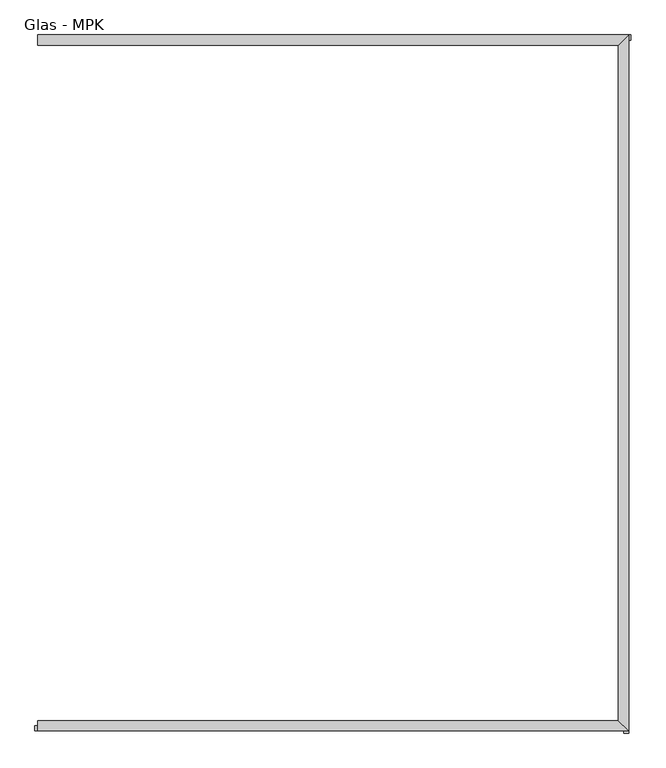
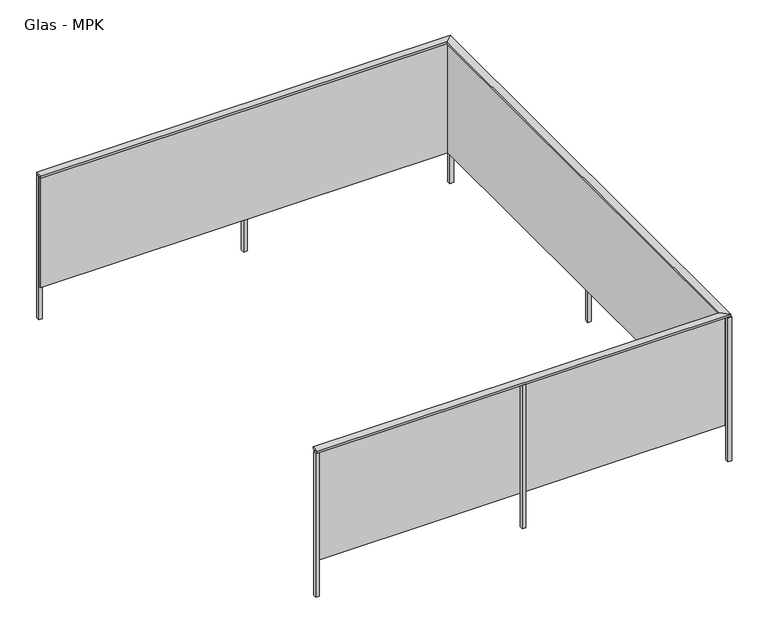
"""IFC4 building model written with IfcOpenShell, lengths in millimetres: railing geometry, Glas - MPK."""

import ifcopenshell
import ifcopenshell.guid

model = None  # the IFC model being written
_history = None  # IfcOwnerHistory: only IFC2X3 demands one
_inside = {}  # id of a spatial element -> (the spatial element, [elements in it])
_under = {}  # id of a project, library or spatial element -> (it, [spatial elements below it])
_declared = {}  # id of a project -> (the project, [libraries it declares])
_typed = {}  # id of a type object -> (the type object, [elements of that type])
_made_of = {}  # id of a material, layer set ... -> (it, [elements and type objects made of it])


def new_model(schema):
    """Start an empty IFC model of exactly this schema.

    Asked for "IFC4X3", IfcOpenShell would pick the latest addendum, in which some entities
    have other attributes; the version numbers below select the first issue.
    IFC2X3 requires an IfcOwnerHistory on every rooted entity: one is made here for all.
    """
    global model, _history
    if schema == "IFC4X3":
        model = ifcopenshell.file(schema_version=(4, 3, 0, 0))
    else:
        model = ifcopenshell.file(schema=schema)
    _inside.clear()
    _under.clear()
    _declared.clear()
    _typed.clear()
    _made_of.clear()
    _history = None
    if model.schema == "IFC2X3":
        org = make("IfcOrganization", Name="unknown")
        user = make(
            "IfcPersonAndOrganization",
            ThePerson=make("IfcPerson", FamilyName="unknown"),
            TheOrganization=org,
        )
        app = make(
            "IfcApplication",
            ApplicationDeveloper=org,
            Version="unknown",
            ApplicationFullName="unknown",
            ApplicationIdentifier="unknown",
        )
        _history = make(
            "IfcOwnerHistory",
            OwningUser=user,
            OwningApplication=app,
            ChangeAction="ADDED",
            CreationDate=0,
        )
    return model


def make(cls, **values):
    """One entity of the class cls with the attributes given. An attribute that is None is left unset."""
    return model.create_entity(
        cls, **{name: value for name, value in values.items() if value is not None}
    )


def rooted(cls, **values):
    """An entity with a GlobalId (a new one), such as an element, a storey or a relation."""
    return make(cls, GlobalId=ifcopenshell.guid.new(), OwnerHistory=_history, **values)


def si_unit(unit_type, name, prefix=None):
    """IfcSIUnit, for example si_unit("LENGTHUNIT", "METRE", prefix="MILLI")."""
    return make("IfcSIUnit", UnitType=unit_type, Prefix=prefix, Name=name)


def assignment(units):
    """IfcUnitAssignment: the units of a project."""
    return None if units is None else make("IfcUnitAssignment", Units=units)


def point(xyz):
    """IfcCartesianPoint."""
    return None if xyz is None else make("IfcCartesianPoint", Coordinates=xyz)


def direction(xyz):
    """IfcDirection."""
    return None if xyz is None else make("IfcDirection", DirectionRatios=xyz)


def frame(location, z_axis=None, x_axis=None):
    """IfcAxis2Placement3D, a coordinate frame: its origin and axes. An axis left out is left unset."""
    return make(
        "IfcAxis2Placement3D",
        Location=point(location),
        Axis=direction(z_axis),
        RefDirection=direction(x_axis),
    )


def origin():
    """The frame at (0, 0, 0) with its axes left unset."""
    return frame((0.0, 0.0, 0.0))


def place(relative_to, where):
    """IfcLocalPlacement: puts the frame where relative to a parent placement (None: the world)."""
    return make(
        "IfcLocalPlacement", PlacementRelTo=relative_to, RelativePlacement=where
    )


def context(
    kind, dimensions, precision=None, world=None, true_north=None, identifier=None
):
    """IfcGeometricRepresentationContext, for example the 3D "Model" context."""
    return make(
        "IfcGeometricRepresentationContext",
        ContextIdentifier=identifier,
        ContextType=kind,
        CoordinateSpaceDimension=dimensions,
        Precision=precision,
        WorldCoordinateSystem=world,
        TrueNorth=true_north,
    )


def project(units=None, contexts=None):
    """IfcProject with its units and contexts."""
    return rooted(
        "IfcProject",
        Name="project",
        RepresentationContexts=contexts,
        UnitsInContext=assignment(units),
    )


def spatial(cls, under=None, at=None, **own):
    """A site, building, storey or space (cls), placed at a placement, below another one or the project."""
    s = rooted(cls, ObjectPlacement=at, **own)
    if under is not None:
        _under.setdefault(under.id(), (under, []))[1].append(s)
    return s


def polyline(points):
    """IfcPolyline through the points."""
    return make("IfcPolyline", Points=[point(p) for p in points])


def outline(outer, holes=None, kind="AREA"):
    """IfcArbitraryClosedProfileDef: a profile drawn as a closed curve; with holes, ...WithVoids."""
    if holes is None:
        return make("IfcArbitraryClosedProfileDef", ProfileType=kind, OuterCurve=outer)
    return make(
        "IfcArbitraryProfileDefWithVoids",
        ProfileType=kind,
        OuterCurve=outer,
        InnerCurves=holes,
    )


def extrude(swept, where, along, depth):
    """IfcExtrudedAreaSolid: the profile swept, set in the frame where, extruded along a direction by depth."""
    return make(
        "IfcExtrudedAreaSolid",
        SweptArea=swept,
        Position=where,
        ExtrudedDirection=direction(along),
        Depth=depth,
    )


def faces_of(points, faces, orient=None, outer=None):
    """IfcFace entities. A face is a list of loops; a loop is a list of indices into points, from 0.

    orient and outer hold one flag for each loop. By default every Orientation is true, the
    first loop of a face is its IfcFaceOuterBound and the others are IfcFaceBound.
    """
    made = []
    for i, loops in enumerate(faces):
        bounds = []
        for j, loop in enumerate(loops):
            is_outer = j == 0 if outer is None else outer[i][j]
            bounds.append(
                make(
                    "IfcFaceOuterBound" if is_outer else "IfcFaceBound",
                    Bound=make("IfcPolyLoop", Polygon=[points[k] for k in loop]),
                    Orientation=True if orient is None else orient[i][j],
                )
            )
        made.append(make("IfcFace", Bounds=bounds))
    return made


def faceted_brep(points, faces, orient=None, outer=None, voids=None):
    """IfcFacetedBrep: a solid bounded by flat faces; with voids (closed shells), ...WithVoids."""
    shared = [point(p) for p in points]
    hull = make("IfcClosedShell", CfsFaces=faces_of(shared, faces, orient, outer))
    if voids is None:
        return make("IfcFacetedBrep", Outer=hull)
    return make(
        "IfcFacetedBrepWithVoids",
        Outer=hull,
        Voids=[
            make(cls, CfsFaces=faces_of(shared, fs, o, b)) for cls, fs, o, b in voids
        ],
    )


def shape(context_of_items, identifier, shape_type, items):
    """IfcShapeRepresentation: the items that make up one representation, for example the "Body"."""
    return make(
        "IfcShapeRepresentation",
        ContextOfItems=context_of_items,
        RepresentationIdentifier=identifier,
        RepresentationType=shape_type,
        Items=items,
    )


def source(mapping_origin, context_of_items, identifier, shape_type, items):
    """IfcRepresentationMap: a shape defined once, which mapped items show again and again."""
    return make(
        "IfcRepresentationMap",
        MappingOrigin=mapping_origin,
        MappedRepresentation=shape(context_of_items, identifier, shape_type, items),
    )


def transform(
    local_origin,
    x_axis=None,
    y_axis=None,
    z_axis=None,
    scale=None,
    scale2=None,
    scale3=None,
    uniform=True,
):
    """IfcCartesianTransformationOperator3D, or its non-uniform kind. x_axis, y_axis, z_axis: its Axis1, 2, 3."""
    if uniform:
        return make(
            "IfcCartesianTransformationOperator3D",
            Axis1=direction(x_axis),
            Axis2=direction(y_axis),
            LocalOrigin=point(local_origin),
            Scale=scale,
            Axis3=direction(z_axis),
        )
    return make(
        "IfcCartesianTransformationOperator3DnonUniform",
        Axis1=direction(x_axis),
        Axis2=direction(y_axis),
        LocalOrigin=point(local_origin),
        Scale=scale,
        Axis3=direction(z_axis),
        Scale2=scale2,
        Scale3=scale3,
    )


def mapped(mapping_source, mapping_target):
    """IfcMappedItem: shows the shape of a source again, moved by a transform."""
    return make(
        "IfcMappedItem", MappingSource=mapping_source, MappingTarget=mapping_target
    )


def made_of(thing, what):
    """Note that an element or type object is made of a material, layer set ...; save() writes the relation."""
    if what is not None:
        _made_of.setdefault(what.id(), (what, []))[1].append(thing)
    return thing


def element(
    cls,
    number,
    at=None,
    inside=None,
    cuts=None,
    type_object=None,
    material=None,
    context=None,
    identifier="Body",
    shape_type=None,
    held_by="IfcProductDefinitionShape",
    body=None,
    shapes=None,
    **own,
):
    """One element of the class cls, such as IfcWall. Its Tag is "e" and its number.

    at: its placement. inside: the storey or other place that contains it. cuts: it is an
    opening in that element (IfcRelVoidsElement). A single representation is given by context,
    identifier, shape_type and body (its items); several are given by shapes. held_by: the class
    of the entity that holds the representations. save() writes the other relations.
    """
    e = rooted(cls, Tag="e%d" % number, ObjectPlacement=at, **own)
    if body is not None:
        shapes = [shape(context, identifier, shape_type, body)]
    if shapes is not None:
        e.Representation = make(held_by, Representations=shapes)
    if inside is not None:
        _inside.setdefault(inside.id(), (inside, []))[1].append(e)
    if cuts is not None:
        rooted(
            "IfcRelVoidsElement", RelatingBuildingElement=cuts, RelatedOpeningElement=e
        )
    if type_object is not None:
        _typed.setdefault(type_object.id(), (type_object, []))[1].append(e)
    return made_of(e, material)


def aggregate(whole, parts):
    """IfcRelAggregates: a whole, such as a stair, and the parts it consists of."""
    return rooted("IfcRelAggregates", RelatingObject=whole, RelatedObjects=parts)


def save(model, path):
    """Write the relations noted so far, then the file.

    IfcRelAggregates (storeys below a building ...), IfcRelContainedInSpatialStructure (elements
    in a storey), IfcRelDefinesByType, IfcRelAssociatesMaterial and IfcRelDeclares: one each for
    every whole, place, type object, material and project.
    """
    for whole, parts in _under.values():
        aggregate(whole, parts)
    for where, things in _inside.values():
        rooted(
            "IfcRelContainedInSpatialStructure",
            RelatedElements=things,
            RelatingStructure=where,
        )
    for kind, things in _typed.values():
        rooted("IfcRelDefinesByType", RelatedObjects=things, RelatingType=kind)
    for what, things in _made_of.values():
        rooted("IfcRelAssociatesMaterial", RelatedObjects=things, RelatingMaterial=what)
    for by, libraries in _declared.values():
        rooted("IfcRelDeclares", RelatingContext=by, RelatedDefinitions=libraries)
    model.write(path)


def glas_mpk_39525c5c(model_context):
    return source(origin(), model_context, "Body", "SolidModel", [
        faceted_brep([(28810.8437289, 1285.374085, 9843.2628643), (28810.8437289, 1235.374085, 9843.2628643), (28810.8437289, 1235.374085, 9856.7371357), (28810.8437289, 1285.374085, 9856.7371357), (31650.8437289, 1285.374085, 9843.2628643), (31600.8437289, 1235.374085, 9843.2628643), (31600.8437289, 1235.374085, 9856.7371357), (31650.8437289, 1285.374085, 9856.7371357), (31650.8437289, -2055.3552612, 9843.2628643), (31600.8437289, -2005.3552612, 9843.2628643), (31600.8437289, -2005.3552612, 9856.7371357), (31650.8437289, -2055.3552612, 9856.7371357), (28810.8437289, -2055.3552612, 9843.2628643), (28810.8437289, -2055.3552612, 9856.7371357), (28810.8437289, -2005.3552612, 9856.7371357), (28810.8437289, -2005.3552612, 9843.2628643)], [[[0, 1, 2, 3]], [[1, 0, 4, 5]], [[2, 1, 5, 6]], [[3, 2, 6, 7]], [[0, 3, 7, 4]], [[5, 4, 8, 9]], [[6, 5, 9, 10]], [[7, 6, 10, 11]], [[4, 7, 11, 8]], [[12, 13, 14, 15]], [[9, 8, 12, 15]], [[10, 9, 15, 14]], [[11, 10, 14, 13]], [[8, 11, 13, 12]]]),
        faceted_brep([(28810.8437289, 1245.374085, 9842.8769824), (28810.8437289, 1259.566209, 9842.8769824), (28810.8437289, 1259.566209, 9042.8769824), (28810.8437289, 1245.374085, 9042.8769824), (31610.8437289, 1245.374085, 9842.8769824), (31625.0358529, 1259.566209, 9842.8769824), (31625.0358529, 1259.566209, 9042.8769824), (31610.8437289, 1245.374085, 9042.8769824), (31610.8437289, -2015.3552612, 9842.8769824), (31625.0358529, -2029.5473852, 9842.8769824), (31625.0358529, -2029.5473852, 9042.8769824), (31610.8437289, -2015.3552612, 9042.8769824), (28810.8437289, -2015.3552612, 9842.8769824), (28810.8437289, -2015.3552612, 9042.8769824), (28810.8437289, -2029.5473852, 9042.8769824), (28810.8437289, -2029.5473852, 9842.8769824)], [[[0, 1, 2, 3]], [[1, 0, 4, 5]], [[2, 1, 5, 6]], [[3, 2, 6, 7]], [[0, 3, 7, 4]], [[5, 4, 8, 9]], [[6, 5, 9, 10]], [[7, 6, 10, 11]], [[4, 7, 11, 8]], [[12, 13, 14, 15]], [[9, 8, 12, 15]], [[10, 9, 15, 14]], [[11, 10, 14, 13]], [[8, 11, 13, 12]]]),
        extrude(outline(polyline([(30242.0937289, -2030.3552612), (30242.0937289, -2055.3552612), (30217.0937289, -2055.3552612), (30217.0937289, -2030.3552612), (30242.0937289, -2030.3552612)])), frame((0.0, 0.0, 8800.0), z_axis=(0.0, 0.0, 1.0), x_axis=(1.0, 0.0, 0.0)), (0.0, 0.0, 1.0), 1043.2628643),
        extrude(outline(polyline([(31625.8437289, -372.4905881), (31650.8437289, -372.4905881), (31650.8437289, -397.4905881), (31625.8437289, -397.4905881), (31625.8437289, -372.4905881)])), frame((0.0, 0.0, 8800.0), z_axis=(0.0, 0.0, 1.0), x_axis=(1.0, 0.0, 0.0)), (0.0, 0.0, 1.0), 1043.2628643),
        extrude(outline(polyline([(30217.0937289, 1260.374085), (30217.0937289, 1285.374085), (30242.0937289, 1285.374085), (30242.0937289, 1260.374085), (30217.0937289, 1260.374085)])), frame((0.0, 0.0, 8800.0), z_axis=(0.0, 0.0, 1.0), x_axis=(1.0, 0.0, 0.0)), (0.0, 0.0, 1.0), 1043.2628643),
        extrude(outline(polyline([(31625.8437289, -2040.3552612), (31650.8437289, -2040.3552612), (31650.8437289, -2065.3552612), (31625.8437289, -2065.3552612), (31625.8437289, -2040.3552612)])), frame((0.0, 0.0, 8800.0), z_axis=(0.0, 0.0, 1.0), x_axis=(1.0, 0.0, 0.0)), (0.0, 0.0, 1.0), 1043.2628643),
        extrude(outline(polyline([(31635.8437289, 1260.374085), (31635.8437289, 1285.374085), (31660.8437289, 1285.374085), (31660.8437289, 1260.374085), (31635.8437289, 1260.374085)])), frame((0.0, 0.0, 8800.0), z_axis=(0.0, 0.0, 1.0), x_axis=(1.0, 0.0, 0.0)), (0.0, 0.0, 1.0), 1043.2628643),
        extrude(outline(polyline([(28823.3437289, -2030.3552612), (28823.3437289, -2055.3552612), (28798.3437289, -2055.3552612), (28798.3437289, -2030.3552612), (28823.3437289, -2030.3552612)])), frame((0.0, 0.0, 8800.0), z_axis=(0.0, 0.0, 1.0), x_axis=(1.0, 0.0, 0.0)), (0.0, 0.0, 1.0), 1043.2628643),
        extrude(outline(polyline([(28810.8437289, 1260.374085), (28810.8437289, 1285.374085), (28835.8437289, 1285.374085), (28835.8437289, 1260.374085), (28810.8437289, 1260.374085)])), frame((0.0, 0.0, 8800.0), z_axis=(0.0, 0.0, 1.0), x_axis=(1.0, 0.0, 0.0)), (0.0, 0.0, 1.0), 1043.2628643),
    ])


if __name__ == "__main__":
    model = new_model("IFC4")
    model_context = context("Model", 3, world=origin())
    ifc_project = project(units=[si_unit("LENGTHUNIT", "METRE", prefix="MILLI")], contexts=[model_context])
    site = spatial("IfcSite", under=ifc_project)
    building = spatial("IfcBuilding", under=site)
    placement = place(None, origin())
    glas_mpk_shape = glas_mpk_39525c5c(model_context)
    element("IfcRailing", 1, ObjectType="Glas - MPK", at=placement, inside=building, context=model_context, shape_type="MappedRepresentation", body=[
        mapped(glas_mpk_shape, transform((0.0, 0.0, 0.0), x_axis=(1.0, 0.0, 0.0), y_axis=(0.0, 1.0, 0.0), z_axis=(0.0, 0.0, 1.0))),
    ])
    save(model, "model.ifc")

# Revit data of these elements
# Element 1 (IfcRailing, "Glas - MPK")
#   Materials on its faces: "Metal - Aluminum", "Window - Glass"
# Materials
#   "Metal - Aluminum": class "Unassigned", colour RGB 247 247 247, transparency 0, Comments = "Rendering appearance not upgraded "
#   "Window - Glass": class "Glas", colour RGB 128 128 255, transparency 0.75
